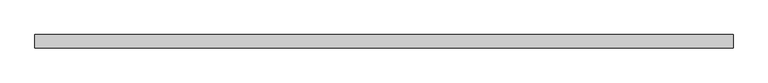
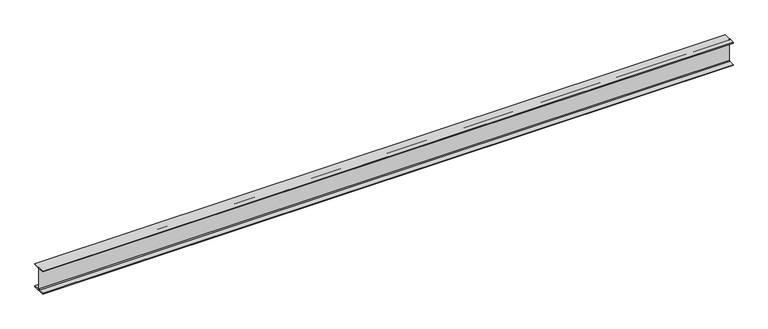
"""IFC4 building model written with IfcOpenShell, lengths in millimetres: beam geometry, Old_Steel Beam_H-KSD3502 : H_SB_ASB_H-300×300x10x15."""

from ifc_helpers import new_model, si_unit, point, frame, frame_2d, origin, place, context, project, spatial, polyline, circle_curve, trimmed, segment, composite_curve, outline, extrude, source, transform, mapped, element, save


def beam_06431c43(model_context):
    return source(origin(), model_context, "Body", "SweptSolid", [
        extrude(outline(composite_curve([segment(polyline([(82.5, -141.5), (82.5, -151.7), (-82.5, -151.7), (-82.5, -141.5), (-11.9, -141.5)]), True, "CONTINUOUS"), segment(trimmed(circle_curve(frame_2d((-11.9, -132.6)), 8.9), [point((-11.9, -141.5))], [point((-3.0, -132.6))], True, "CARTESIAN"), True, "CONTINUOUS"), segment(polyline([(-3.0, -132.6), (-3.0, 132.6)]), True, "CONTINUOUS"), segment(trimmed(circle_curve(frame_2d((-11.9, 132.6)), 8.9), [point((-3.0, 132.6))], [point((-11.9, 141.5))], True, "CARTESIAN"), True, "CONTINUOUS"), segment(polyline([(-11.9, 141.5), (-82.5, 141.5), (-82.5, 151.7), (82.5, 151.7), (82.5, 141.5), (11.9, 141.5)]), True, "CONTINUOUS"), segment(trimmed(circle_curve(frame_2d((11.9, 132.6)), 8.9), [point((11.9, 141.5))], [point((3.0, 132.6))], True, "CARTESIAN"), True, "CONTINUOUS"), segment(polyline([(3.0, 132.6), (3.0, -132.6)]), True, "CONTINUOUS"), segment(trimmed(circle_curve(frame_2d((11.9, -132.6)), 8.9), [point((3.0, -132.6))], [point((11.9, -141.5))], True, "CARTESIAN"), True, "CONTINUOUS"), segment(polyline([(11.9, -141.5), (82.5, -141.5)]), True, "CONTINUOUS")], self_intersect=False)), frame((-4272.9251782, 0.0, 0.0), z_axis=(1.0, 0.0, 0.0), x_axis=(0.0, 1.0, 0.0)), (0.0, 0.0, 1.0), 8647.1704515),
    ])


if __name__ == "__main__":
    model = new_model("IFC4")
    model_context = context("Model", 3, world=origin())
    ifc_project = project(units=[si_unit("LENGTHUNIT", "METRE", prefix="MILLI")], contexts=[model_context])
    site = spatial("IfcSite", under=ifc_project)
    building = spatial("IfcBuilding", under=site)
    placement = place(None, origin())
    beam_shape = beam_06431c43(model_context)
    element("IfcBeam", 1, ObjectType="Old_Steel Beam_H-KSD3502 : H_SB_ASB_H-300×300x10x15", at=placement, inside=building, context=model_context, shape_type="MappedRepresentation", body=[
        mapped(beam_shape, transform((0.0, 0.0, 0.0), x_axis=(1.0, 0.0, 0.0), y_axis=(0.0, 1.0, 0.0), z_axis=(0.0, 0.0, 1.0))),
    ])
    save(model, "model.ifc")

# Revit data of these elements
# Type "Old_Steel Beam_H-KSD3502 : H_SB_ASB_H-300×300x10x15"
#   Width = 30.0 cm
#   Web Thickness = 1.0 cm
#   Web Fillet = 1.8 cm
#   Warping Constant = 1370670.0 cm⁶
#   Torsional Moment of Inertia = 77.00 cm⁴
#   Torsional Modulus = 1.0 cm³
#   Section Area = 119.8 cm²
#   Plastic Modulus weak axis = 684.0 cm³
#   Plastic Modulus strong axis = 1500.0 cm³
#   Perimeter = 1.75 m²/m
#   Nominal Weight = 94.00 kgf/m
#   Moment of Inertia weak axis = 6750.00 cm⁴
#   Moment of Inertia strong axis = 20400.00 cm⁴
#   Height = 30.0 cm
#   Flange Thickness = 1.5 cm
#   Elastic Modulus weak axis = 450.0 cm³
#   Elastic Modulus strong axis = 1360.0 cm³
#   Centroid Vertical = 15.0 cm
#   Centroid Horizontal = 15.0 cm
#   Length [instance default] = 1.5240 m
#   Structural Material [instance default] = Steel, 45-345
#   Assembly Code = ""
# Element 1 (IfcBeam, "Old_Steel Beam_H-KSD3502 : H_SB_ASB_H-300×300x10x15")
#   Structural Material = none
# Materials
#   "Steel, 45-345": class "Metal", colour RGB 189 187 185, transparency 0, Description = "Steel 345 MPa", Cost = 0
